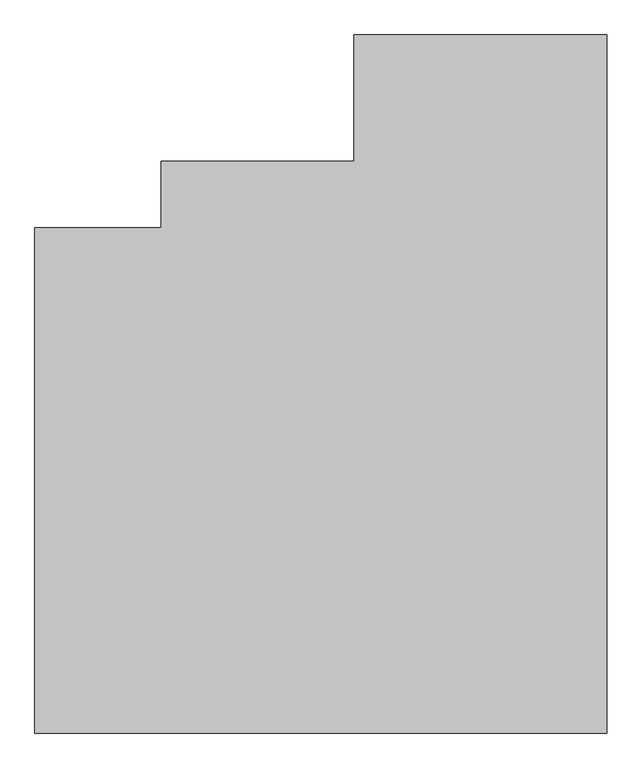
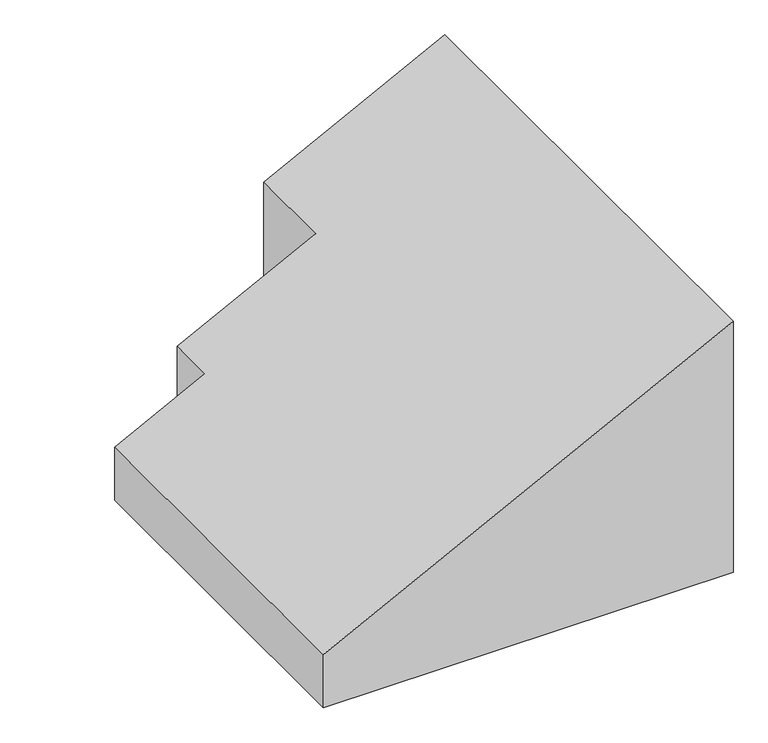
"""IFC4 building model written with IfcOpenShell, lengths in millimetres: proxy geometry, 0_3d."""

import ifcopenshell
import ifcopenshell.guid

model = None  # the IFC model being written
_history = None  # IfcOwnerHistory: only IFC2X3 demands one
_inside = {}  # id of a spatial element -> (the spatial element, [elements in it])
_under = {}  # id of a project, library or spatial element -> (it, [spatial elements below it])
_declared = {}  # id of a project -> (the project, [libraries it declares])
_typed = {}  # id of a type object -> (the type object, [elements of that type])
_made_of = {}  # id of a material, layer set ... -> (it, [elements and type objects made of it])


def new_model(schema):
    """Start an empty IFC model of exactly this schema.

    Asked for "IFC4X3", IfcOpenShell would pick the latest addendum, in which some entities
    have other attributes; the version numbers below select the first issue.
    IFC2X3 requires an IfcOwnerHistory on every rooted entity: one is made here for all.
    """
    global model, _history
    if schema == "IFC4X3":
        model = ifcopenshell.file(schema_version=(4, 3, 0, 0))
    else:
        model = ifcopenshell.file(schema=schema)
    _inside.clear()
    _under.clear()
    _declared.clear()
    _typed.clear()
    _made_of.clear()
    _history = None
    if model.schema == "IFC2X3":
        org = make("IfcOrganization", Name="unknown")
        user = make(
            "IfcPersonAndOrganization",
            ThePerson=make("IfcPerson", FamilyName="unknown"),
            TheOrganization=org,
        )
        app = make(
            "IfcApplication",
            ApplicationDeveloper=org,
            Version="unknown",
            ApplicationFullName="unknown",
            ApplicationIdentifier="unknown",
        )
        _history = make(
            "IfcOwnerHistory",
            OwningUser=user,
            OwningApplication=app,
            ChangeAction="ADDED",
            CreationDate=0,
        )
    return model


def make(cls, **values):
    """One entity of the class cls with the attributes given. An attribute that is None is left unset."""
    return model.create_entity(
        cls, **{name: value for name, value in values.items() if value is not None}
    )


def rooted(cls, **values):
    """An entity with a GlobalId (a new one), such as an element, a storey or a relation."""
    return make(cls, GlobalId=ifcopenshell.guid.new(), OwnerHistory=_history, **values)


def si_unit(unit_type, name, prefix=None):
    """IfcSIUnit, for example si_unit("LENGTHUNIT", "METRE", prefix="MILLI")."""
    return make("IfcSIUnit", UnitType=unit_type, Prefix=prefix, Name=name)


def assignment(units):
    """IfcUnitAssignment: the units of a project."""
    return None if units is None else make("IfcUnitAssignment", Units=units)


def point(xyz):
    """IfcCartesianPoint."""
    return None if xyz is None else make("IfcCartesianPoint", Coordinates=xyz)


def direction(xyz):
    """IfcDirection."""
    return None if xyz is None else make("IfcDirection", DirectionRatios=xyz)


def frame(location, z_axis=None, x_axis=None):
    """IfcAxis2Placement3D, a coordinate frame: its origin and axes. An axis left out is left unset."""
    return make(
        "IfcAxis2Placement3D",
        Location=point(location),
        Axis=direction(z_axis),
        RefDirection=direction(x_axis),
    )


def origin():
    """The frame at (0, 0, 0) with its axes left unset."""
    return frame((0.0, 0.0, 0.0))


def place(relative_to, where):
    """IfcLocalPlacement: puts the frame where relative to a parent placement (None: the world)."""
    return make(
        "IfcLocalPlacement", PlacementRelTo=relative_to, RelativePlacement=where
    )


def context(
    kind, dimensions, precision=None, world=None, true_north=None, identifier=None
):
    """IfcGeometricRepresentationContext, for example the 3D "Model" context."""
    return make(
        "IfcGeometricRepresentationContext",
        ContextIdentifier=identifier,
        ContextType=kind,
        CoordinateSpaceDimension=dimensions,
        Precision=precision,
        WorldCoordinateSystem=world,
        TrueNorth=true_north,
    )


def project(units=None, contexts=None):
    """IfcProject with its units and contexts."""
    return rooted(
        "IfcProject",
        Name="project",
        RepresentationContexts=contexts,
        UnitsInContext=assignment(units),
    )


def spatial(cls, under=None, at=None, **own):
    """A site, building, storey or space (cls), placed at a placement, below another one or the project."""
    s = rooted(cls, ObjectPlacement=at, **own)
    if under is not None:
        _under.setdefault(under.id(), (under, []))[1].append(s)
    return s


def faces_of(points, faces, orient=None, outer=None):
    """IfcFace entities. A face is a list of loops; a loop is a list of indices into points, from 0.

    orient and outer hold one flag for each loop. By default every Orientation is true, the
    first loop of a face is its IfcFaceOuterBound and the others are IfcFaceBound.
    """
    made = []
    for i, loops in enumerate(faces):
        bounds = []
        for j, loop in enumerate(loops):
            is_outer = j == 0 if outer is None else outer[i][j]
            bounds.append(
                make(
                    "IfcFaceOuterBound" if is_outer else "IfcFaceBound",
                    Bound=make("IfcPolyLoop", Polygon=[points[k] for k in loop]),
                    Orientation=True if orient is None else orient[i][j],
                )
            )
        made.append(make("IfcFace", Bounds=bounds))
    return made


def faceted_brep(points, faces, orient=None, outer=None, voids=None):
    """IfcFacetedBrep: a solid bounded by flat faces; with voids (closed shells), ...WithVoids."""
    shared = [point(p) for p in points]
    hull = make("IfcClosedShell", CfsFaces=faces_of(shared, faces, orient, outer))
    if voids is None:
        return make("IfcFacetedBrep", Outer=hull)
    return make(
        "IfcFacetedBrepWithVoids",
        Outer=hull,
        Voids=[
            make(cls, CfsFaces=faces_of(shared, fs, o, b)) for cls, fs, o, b in voids
        ],
    )


def shape(context_of_items, identifier, shape_type, items):
    """IfcShapeRepresentation: the items that make up one representation, for example the "Body"."""
    return make(
        "IfcShapeRepresentation",
        ContextOfItems=context_of_items,
        RepresentationIdentifier=identifier,
        RepresentationType=shape_type,
        Items=items,
    )


def source(mapping_origin, context_of_items, identifier, shape_type, items):
    """IfcRepresentationMap: a shape defined once, which mapped items show again and again."""
    return make(
        "IfcRepresentationMap",
        MappingOrigin=mapping_origin,
        MappedRepresentation=shape(context_of_items, identifier, shape_type, items),
    )


def transform(
    local_origin,
    x_axis=None,
    y_axis=None,
    z_axis=None,
    scale=None,
    scale2=None,
    scale3=None,
    uniform=True,
):
    """IfcCartesianTransformationOperator3D, or its non-uniform kind. x_axis, y_axis, z_axis: its Axis1, 2, 3."""
    if uniform:
        return make(
            "IfcCartesianTransformationOperator3D",
            Axis1=direction(x_axis),
            Axis2=direction(y_axis),
            LocalOrigin=point(local_origin),
            Scale=scale,
            Axis3=direction(z_axis),
        )
    return make(
        "IfcCartesianTransformationOperator3DnonUniform",
        Axis1=direction(x_axis),
        Axis2=direction(y_axis),
        LocalOrigin=point(local_origin),
        Scale=scale,
        Axis3=direction(z_axis),
        Scale2=scale2,
        Scale3=scale3,
    )


def mapped(mapping_source, mapping_target):
    """IfcMappedItem: shows the shape of a source again, moved by a transform."""
    return make(
        "IfcMappedItem", MappingSource=mapping_source, MappingTarget=mapping_target
    )


def made_of(thing, what):
    """Note that an element or type object is made of a material, layer set ...; save() writes the relation."""
    if what is not None:
        _made_of.setdefault(what.id(), (what, []))[1].append(thing)
    return thing


def element(
    cls,
    number,
    at=None,
    inside=None,
    cuts=None,
    type_object=None,
    material=None,
    context=None,
    identifier="Body",
    shape_type=None,
    held_by="IfcProductDefinitionShape",
    body=None,
    shapes=None,
    **own,
):
    """One element of the class cls, such as IfcWall. Its Tag is "e" and its number.

    at: its placement. inside: the storey or other place that contains it. cuts: it is an
    opening in that element (IfcRelVoidsElement). A single representation is given by context,
    identifier, shape_type and body (its items); several are given by shapes. held_by: the class
    of the entity that holds the representations. save() writes the other relations.
    """
    e = rooted(cls, Tag="e%d" % number, ObjectPlacement=at, **own)
    if body is not None:
        shapes = [shape(context, identifier, shape_type, body)]
    if shapes is not None:
        e.Representation = make(held_by, Representations=shapes)
    if inside is not None:
        _inside.setdefault(inside.id(), (inside, []))[1].append(e)
    if cuts is not None:
        rooted(
            "IfcRelVoidsElement", RelatingBuildingElement=cuts, RelatedOpeningElement=e
        )
    if type_object is not None:
        _typed.setdefault(type_object.id(), (type_object, []))[1].append(e)
    return made_of(e, material)


def aggregate(whole, parts):
    """IfcRelAggregates: a whole, such as a stair, and the parts it consists of."""
    return rooted("IfcRelAggregates", RelatingObject=whole, RelatedObjects=parts)


def save(model, path):
    """Write the relations noted so far, then the file.

    IfcRelAggregates (storeys below a building ...), IfcRelContainedInSpatialStructure (elements
    in a storey), IfcRelDefinesByType, IfcRelAssociatesMaterial and IfcRelDeclares: one each for
    every whole, place, type object, material and project.
    """
    for whole, parts in _under.values():
        aggregate(whole, parts)
    for where, things in _inside.values():
        rooted(
            "IfcRelContainedInSpatialStructure",
            RelatedElements=things,
            RelatingStructure=where,
        )
    for kind, things in _typed.values():
        rooted("IfcRelDefinesByType", RelatedObjects=things, RelatingType=kind)
    for what, things in _made_of.values():
        rooted("IfcRelAssociatesMaterial", RelatedObjects=things, RelatingMaterial=what)
    for by, libraries in _declared.values():
        rooted("IfcRelDeclares", RelatingContext=by, RelatedDefinitions=libraries)
    model.write(path)


def generic_models_4c10badf(model_context):
    return source(origin(), model_context, "Body", "Brep", [
        faceted_brep([(4650.0, 5670.0, 3007.913011), (2595.0, 5670.0, 1960.8382122), (2595.0, 4645.0, 1960.8382122), (1025.0, 4645.0, 1160.8832565), (1025.0, 4105.0, 1160.8832565), (0.0, 4105.0, 638.6196708), (0.0, 0.0, 638.6196708), (4650.0, 0.0, 3007.913011), (1025.0, 4105.0, 0.0), (0.0, 4105.0, 0.0), (1025.0, 4645.0, 0.0), (2595.0, 4645.0, 0.0), (2595.0, 5670.0, 0.0), (4650.0, 5670.0, 0.0), (4650.0, 0.0, 0.0), (0.0, 0.0, 0.0)], [[[0, 1, 2, 3, 4, 5, 6, 7]], [[5, 4, 8, 9]], [[4, 3, 10, 8]], [[3, 2, 11, 10]], [[2, 1, 12, 11]], [[1, 0, 13, 12]], [[14, 13, 0, 7]], [[7, 6, 15, 14]], [[6, 5, 9, 15]], [[11, 12, 13, 14, 15, 9, 8, 10]]]),
    ])


if __name__ == "__main__":
    model = new_model("IFC4")
    model_context = context("Model", 3, world=origin())
    ifc_project = project(units=[si_unit("LENGTHUNIT", "METRE", prefix="MILLI")], contexts=[model_context])
    site = spatial("IfcSite", under=ifc_project)
    building = spatial("IfcBuilding", under=site)
    placement = place(None, origin())
    generic_models_shape = generic_models_4c10badf(model_context)
    element("IfcBuildingElementProxy", 1, Name="0_3d", ObjectType="0_3d", at=placement, inside=building, context=model_context, shape_type="MappedRepresentation", body=[
        mapped(generic_models_shape, transform((0.0, 0.0, 0.0), x_axis=(1.0, 0.0, 0.0), y_axis=(0.0, 1.0, 0.0), z_axis=(0.0, 0.0, 1.0))),
    ])
    save(model, "model.ifc")

# Revit data of these elements
# Element 1 (IfcBuildingElementProxy, "0_3d")
#   Materials on its faces: "*1"
# Materials
#   "*1": class "Unassigned", colour RGB 175 175 175, transparency 0
